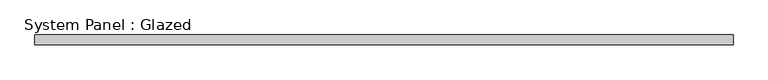
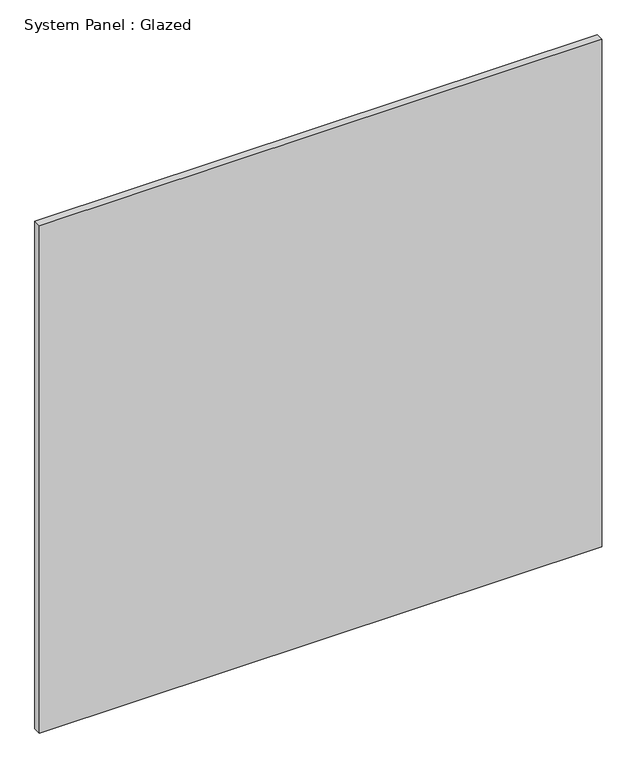
"""IFC4 building model written with IfcOpenShell, lengths in millimetres: plate geometry, System Panel : Glazed."""

from ifc_helpers import new_model, si_unit, origin, origin_with_axes, place, context, project, spatial, polyline, outline, extrude, source, transform, mapped, element, save


def system_panel_glazed_c3495617(model_context):
    return source(origin(), model_context, "Body", "SweptSolid", [
        extrude(outline(polyline([(902.5000002, 24.5), (-902.5000002, 24.5), (-902.5000002, 49.5), (902.5000002, 49.5), (902.5000002, 24.5)])), origin_with_axes(), (0.0, 0.0, 1.0), 1722.3836314),
    ])


if __name__ == "__main__":
    model = new_model("IFC4")
    model_context = context("Model", 3, world=origin())
    ifc_project = project(units=[si_unit("LENGTHUNIT", "METRE", prefix="MILLI")], contexts=[model_context])
    site = spatial("IfcSite", under=ifc_project)
    building = spatial("IfcBuilding", under=site)
    placement = place(None, origin())
    system_panel_glazed_shape = system_panel_glazed_c3495617(model_context)
    element("IfcPlate", 1, ObjectType="System Panel : Glazed", at=placement, inside=building, context=model_context, shape_type="MappedRepresentation", body=[
        mapped(system_panel_glazed_shape, transform((0.0, 0.0, 0.0), x_axis=(1.0, 0.0, 0.0), y_axis=(0.0, 1.0, 0.0), z_axis=(0.0, 0.0, 1.0))),
    ])
    save(model, "model.ifc")

# Revit data of these elements
# Element 1 (IfcPlate, "System Panel : Glazed")
#   Materials on its faces: "Glass"
# Materials
#   "Glass": class "Glass", colour RGB 218 227 224, transparency 0.85, Description = "Soda Lime Glass", Cost = 0
